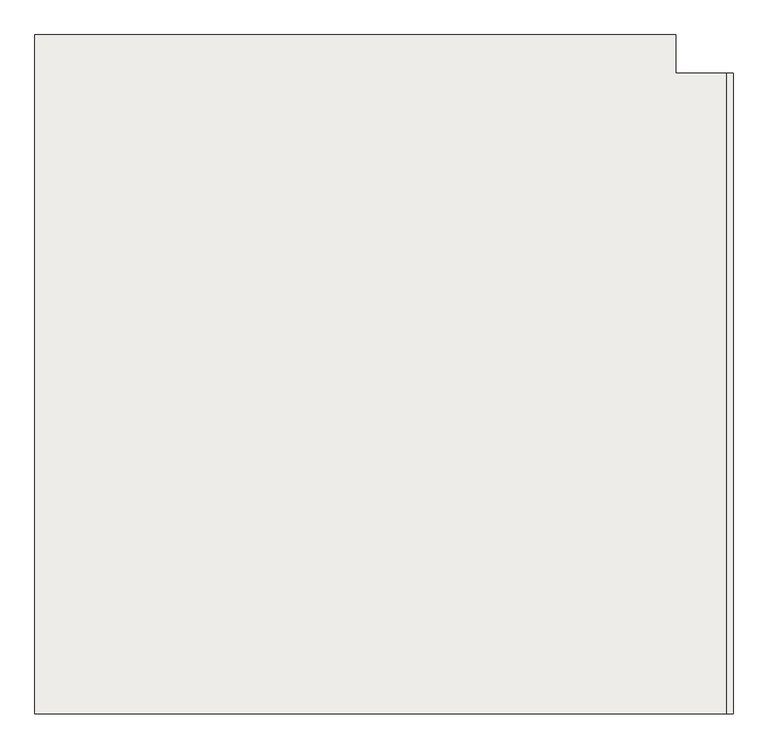
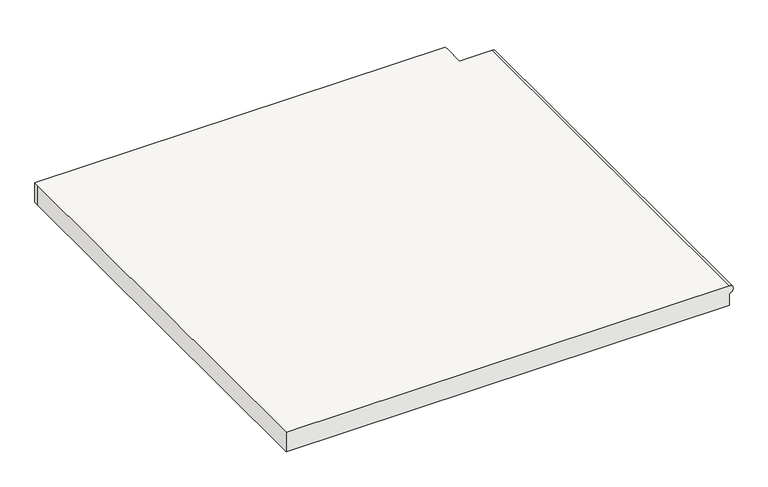
"""IFC4 building model written with IfcOpenShell, lengths in millimetres: slab geometry."""

import ifcopenshell
import ifcopenshell.guid

model = None  # the IFC model being written
_history = None  # IfcOwnerHistory: only IFC2X3 demands one
_inside = {}  # id of a spatial element -> (the spatial element, [elements in it])
_under = {}  # id of a project, library or spatial element -> (it, [spatial elements below it])
_declared = {}  # id of a project -> (the project, [libraries it declares])
_typed = {}  # id of a type object -> (the type object, [elements of that type])
_made_of = {}  # id of a material, layer set ... -> (it, [elements and type objects made of it])


def new_model(schema):
    """Start an empty IFC model of exactly this schema.

    Asked for "IFC4X3", IfcOpenShell would pick the latest addendum, in which some entities
    have other attributes; the version numbers below select the first issue.
    IFC2X3 requires an IfcOwnerHistory on every rooted entity: one is made here for all.
    """
    global model, _history
    if schema == "IFC4X3":
        model = ifcopenshell.file(schema_version=(4, 3, 0, 0))
    else:
        model = ifcopenshell.file(schema=schema)
    _inside.clear()
    _under.clear()
    _declared.clear()
    _typed.clear()
    _made_of.clear()
    _history = None
    if model.schema == "IFC2X3":
        org = make("IfcOrganization", Name="unknown")
        user = make(
            "IfcPersonAndOrganization",
            ThePerson=make("IfcPerson", FamilyName="unknown"),
            TheOrganization=org,
        )
        app = make(
            "IfcApplication",
            ApplicationDeveloper=org,
            Version="unknown",
            ApplicationFullName="unknown",
            ApplicationIdentifier="unknown",
        )
        _history = make(
            "IfcOwnerHistory",
            OwningUser=user,
            OwningApplication=app,
            ChangeAction="ADDED",
            CreationDate=0,
        )
    return model


def make(cls, **values):
    """One entity of the class cls with the attributes given. An attribute that is None is left unset."""
    return model.create_entity(
        cls, **{name: value for name, value in values.items() if value is not None}
    )


def rooted(cls, **values):
    """An entity with a GlobalId (a new one), such as an element, a storey or a relation."""
    return make(cls, GlobalId=ifcopenshell.guid.new(), OwnerHistory=_history, **values)


def si_unit(unit_type, name, prefix=None):
    """IfcSIUnit, for example si_unit("LENGTHUNIT", "METRE", prefix="MILLI")."""
    return make("IfcSIUnit", UnitType=unit_type, Prefix=prefix, Name=name)


def assignment(units):
    """IfcUnitAssignment: the units of a project."""
    return None if units is None else make("IfcUnitAssignment", Units=units)


def point(xyz):
    """IfcCartesianPoint."""
    return None if xyz is None else make("IfcCartesianPoint", Coordinates=xyz)


def direction(xyz):
    """IfcDirection."""
    return None if xyz is None else make("IfcDirection", DirectionRatios=xyz)


def frame(location, z_axis=None, x_axis=None):
    """IfcAxis2Placement3D, a coordinate frame: its origin and axes. An axis left out is left unset."""
    return make(
        "IfcAxis2Placement3D",
        Location=point(location),
        Axis=direction(z_axis),
        RefDirection=direction(x_axis),
    )


def origin():
    """The frame at (0, 0, 0) with its axes left unset."""
    return frame((0.0, 0.0, 0.0))


def place(relative_to, where):
    """IfcLocalPlacement: puts the frame where relative to a parent placement (None: the world)."""
    return make(
        "IfcLocalPlacement", PlacementRelTo=relative_to, RelativePlacement=where
    )


def context(
    kind, dimensions, precision=None, world=None, true_north=None, identifier=None
):
    """IfcGeometricRepresentationContext, for example the 3D "Model" context."""
    return make(
        "IfcGeometricRepresentationContext",
        ContextIdentifier=identifier,
        ContextType=kind,
        CoordinateSpaceDimension=dimensions,
        Precision=precision,
        WorldCoordinateSystem=world,
        TrueNorth=true_north,
    )


def project(units=None, contexts=None):
    """IfcProject with its units and contexts."""
    return rooted(
        "IfcProject",
        Name="project",
        RepresentationContexts=contexts,
        UnitsInContext=assignment(units),
    )


def spatial(cls, under=None, at=None, **own):
    """A site, building, storey or space (cls), placed at a placement, below another one or the project."""
    s = rooted(cls, ObjectPlacement=at, **own)
    if under is not None:
        _under.setdefault(under.id(), (under, []))[1].append(s)
    return s


def circle_curve(where, radius):
    """IfcCircle in the frame where."""
    return make("IfcCircle", Position=where, Radius=radius)


def shape(context_of_items, identifier, shape_type, items):
    """IfcShapeRepresentation: the items that make up one representation, for example the "Body"."""
    return make(
        "IfcShapeRepresentation",
        ContextOfItems=context_of_items,
        RepresentationIdentifier=identifier,
        RepresentationType=shape_type,
        Items=items,
    )


def source(mapping_origin, context_of_items, identifier, shape_type, items):
    """IfcRepresentationMap: a shape defined once, which mapped items show again and again."""
    return make(
        "IfcRepresentationMap",
        MappingOrigin=mapping_origin,
        MappedRepresentation=shape(context_of_items, identifier, shape_type, items),
    )


def transform(
    local_origin,
    x_axis=None,
    y_axis=None,
    z_axis=None,
    scale=None,
    scale2=None,
    scale3=None,
    uniform=True,
):
    """IfcCartesianTransformationOperator3D, or its non-uniform kind. x_axis, y_axis, z_axis: its Axis1, 2, 3."""
    if uniform:
        return make(
            "IfcCartesianTransformationOperator3D",
            Axis1=direction(x_axis),
            Axis2=direction(y_axis),
            LocalOrigin=point(local_origin),
            Scale=scale,
            Axis3=direction(z_axis),
        )
    return make(
        "IfcCartesianTransformationOperator3DnonUniform",
        Axis1=direction(x_axis),
        Axis2=direction(y_axis),
        LocalOrigin=point(local_origin),
        Scale=scale,
        Axis3=direction(z_axis),
        Scale2=scale2,
        Scale3=scale3,
    )


def mapped(mapping_source, mapping_target):
    """IfcMappedItem: shows the shape of a source again, moved by a transform."""
    return make(
        "IfcMappedItem", MappingSource=mapping_source, MappingTarget=mapping_target
    )


def made_of(thing, what):
    """Note that an element or type object is made of a material, layer set ...; save() writes the relation."""
    if what is not None:
        _made_of.setdefault(what.id(), (what, []))[1].append(thing)
    return thing


def element(
    cls,
    number,
    at=None,
    inside=None,
    cuts=None,
    type_object=None,
    material=None,
    context=None,
    identifier="Body",
    shape_type=None,
    held_by="IfcProductDefinitionShape",
    body=None,
    shapes=None,
    **own,
):
    """One element of the class cls, such as IfcWall. Its Tag is "e" and its number.

    at: its placement. inside: the storey or other place that contains it. cuts: it is an
    opening in that element (IfcRelVoidsElement). A single representation is given by context,
    identifier, shape_type and body (its items); several are given by shapes. held_by: the class
    of the entity that holds the representations. save() writes the other relations.
    """
    e = rooted(cls, Tag="e%d" % number, ObjectPlacement=at, **own)
    if body is not None:
        shapes = [shape(context, identifier, shape_type, body)]
    if shapes is not None:
        e.Representation = make(held_by, Representations=shapes)
    if inside is not None:
        _inside.setdefault(inside.id(), (inside, []))[1].append(e)
    if cuts is not None:
        rooted(
            "IfcRelVoidsElement", RelatingBuildingElement=cuts, RelatedOpeningElement=e
        )
    if type_object is not None:
        _typed.setdefault(type_object.id(), (type_object, []))[1].append(e)
    return made_of(e, material)


def aggregate(whole, parts):
    """IfcRelAggregates: a whole, such as a stair, and the parts it consists of."""
    return rooted("IfcRelAggregates", RelatingObject=whole, RelatedObjects=parts)


def save(model, path):
    """Write the relations noted so far, then the file.

    IfcRelAggregates (storeys below a building ...), IfcRelContainedInSpatialStructure (elements
    in a storey), IfcRelDefinesByType, IfcRelAssociatesMaterial and IfcRelDeclares: one each for
    every whole, place, type object, material and project.
    """
    for whole, parts in _under.values():
        aggregate(whole, parts)
    for where, things in _inside.values():
        rooted(
            "IfcRelContainedInSpatialStructure",
            RelatedElements=things,
            RelatingStructure=where,
        )
    for kind, things in _typed.values():
        rooted("IfcRelDefinesByType", RelatedObjects=things, RelatingType=kind)
    for what, things in _made_of.values():
        rooted("IfcRelAssociatesMaterial", RelatedObjects=things, RelatingMaterial=what)
    for by, libraries in _declared.values():
        rooted("IfcRelDeclares", RelatingContext=by, RelatedDefinitions=libraries)
    model.write(path)


def plane_surface(at):
    """IfcPlane: the flat surface through the origin of the frame at, square to its z axis."""
    return make("IfcPlane", Position=at)


def cylinder_surface(at, radius):
    """IfcCylindricalSurface: all points at the distance radius from the z axis of the frame at."""
    return make("IfcCylindricalSurface", Position=at, Radius=radius)


def advanced_brep(points, edges, surfaces, faces):
    """IfcAdvancedBrep: a solid bounded by faces that lie on surfaces and meet in shared edges.

    An edge is (start, end): straight between two places in points (the first is 0);
    or (start, end, curve); or (start, end, curve, False) where it runs against its curve.
    A face is (place in surfaces, loops), or (place, loops, False) where it looks against
    its surface's normal. A loop lists edges by number (the first is 1), with a minus sign
    where the edge is run from its end to its start. The first loop is the outer one.
    """
    corners = [point(p) for p in points]
    vertices = [make("IfcVertexPoint", VertexGeometry=c) for c in corners]
    made = []
    for start, end, *more in edges:
        made.append(
            make(
                "IfcEdgeCurve",
                EdgeStart=vertices[start],
                EdgeEnd=vertices[end],
                EdgeGeometry=more[0] if more else make("IfcPolyline", Points=[corners[start], corners[end]]),
                SameSense=more[1] if len(more) > 1 else True,
            )
        )
    hull = []
    for where, loops, *sense in faces:
        bounds = []
        for j, loop in enumerate(loops):
            ring = [make("IfcOrientedEdge", EdgeElement=made[abs(k) - 1], Orientation=k > 0) for k in loop]
            bounds.append(
                make(
                    "IfcFaceOuterBound" if j == 0 else "IfcFaceBound",
                    Bound=make("IfcEdgeLoop", EdgeList=ring),
                    Orientation=True,
                )
            )
        hull.append(make("IfcAdvancedFace", Bounds=bounds, FaceSurface=surfaces[where], SameSense=sense[0] if sense else True))
    return make("IfcAdvancedBrep", Outer=make("IfcClosedShell", CfsFaces=hull))


def slab_10a918a9(model_context):
    return source(origin(), model_context, "Body", "AdvancedBrep", [
        advanced_brep(
        [(-2595.8194784, -2645.3813072, 638.8235294), (-2595.8194784, -2645.3813072, 658.8235294), (-2595.8194784, -3645.3813072, 658.8235294), (-2595.8194784, -3645.3813072, 638.8235294), (-2675.5365014, -2645.3813072, 658.8235294), (-2675.5365014, -2595.3813072, 658.8235294), (-2675.5365014, -2585.3813072, 658.8235294), (-3675.5365014, -2585.3813072, 658.8235294), (-3675.5365014, -2595.3813072, 658.8235294), (-3675.5365014, -3645.3813072, 658.8235294), (-2595.8194784, -2645.3813072, 608.8235294), (-2595.8194784, -3645.3813072, 608.8235294), (-3675.5365014, -3645.3813072, 608.8235294), (-3675.5365014, -2595.3813072, 608.8235294), (-3675.5365014, -2585.3813072, 608.8235294), (-2675.5365014, -2585.3813072, 608.8235294), (-2675.5365014, -2595.3813072, 608.8235294), (-2675.5365014, -2645.3813072, 608.8235294)],
        [
            (0, 1, circle_curve(frame((-2595.8194784, -2645.3813072, 648.8235294), z_axis=(0.0, -1.0, 0.0), x_axis=(-1.0, 0.0, 0.0)), 10.0)),
            (1, 2),
            (2, 3, circle_curve(frame((-2595.8194784, -3645.3813072, 648.8235294), z_axis=(0.0, 1.0, 0.0), x_axis=(-1.0, 0.0, 0.0)), 10.0)),
            (3, 0),
            (1, 4),
            (4, 5),
            (5, 6),
            (6, 7),
            (7, 8),
            (8, 9),
            (9, 2),
            (10, 11),
            (11, 12),
            (12, 13),
            (13, 14),
            (14, 15),
            (15, 16),
            (16, 17),
            (17, 10),
            (10, 0),
            (3, 11),
            (17, 4),
            (16, 5),
            (15, 6),
            (14, 7),
            (13, 8),
            (12, 9),
        ],
        [
            cylinder_surface(frame((-2595.8194784, -2645.3813072, 648.8235294), z_axis=(0.0, 1.0, 0.0), x_axis=(-1.0, 0.0, 0.0)), 10.0),
            plane_surface(frame((-2595.8194784, -3645.3813072, 658.8235294), z_axis=(0.0, 0.0, 1.0), x_axis=(0.0, 1.0, 0.0))),
            plane_surface(frame((-2595.8194784, -3645.3813072, 608.8235294), z_axis=(0.0, 0.0, -1.0), x_axis=(0.0, -1.0, 0.0))),
            plane_surface(frame((-2595.8194784, -3645.3813072, 658.8235294), z_axis=(1.0, 0.0, 0.0), x_axis=(0.0, 0.0, -1.0))),
            plane_surface(frame((-2595.8194784, -2645.3813072, 658.8235294), z_axis=(0.0, 1.0, 0.0), x_axis=(0.0, 0.0, -1.0))),
            plane_surface(frame((-2675.5365014, -2645.3813072, 658.8235294), z_axis=(1.0, 0.0, 0.0), x_axis=(0.0, 0.0, -1.0))),
            plane_surface(frame((-2675.5365014, -2595.3813072, 658.8235294), z_axis=(1.0, 0.0, 0.0), x_axis=(0.0, 0.0, -1.0))),
            plane_surface(frame((-2675.5365014, -2585.3813072, 658.8235294), z_axis=(0.0, 1.0, 0.0), x_axis=(0.0, 0.0, -1.0))),
            plane_surface(frame((-3675.5365014, -2585.3813072, 658.8235294), z_axis=(-1.0, 0.0, 0.0), x_axis=(0.0, 0.0, -1.0))),
            plane_surface(frame((-3675.5365014, -2595.3813072, 658.8235294), z_axis=(-1.0, 0.0, 0.0), x_axis=(0.0, 0.0, -1.0))),
            plane_surface(frame((-3675.5365014, -3645.3813072, 658.8235294), z_axis=(0.0, -1.0, 0.0), x_axis=(0.0, 0.0, -1.0))),
        ],
        [
            (0, [[1, 2, 3, 4]]),
            (1, [[5, 6, 7, 8, 9, 10, 11, -2]]),
            (2, [[12, 13, 14, 15, 16, 17, 18, 19]]),
            (3, [[-12, 20, -4, 21]]),
            (4, [[-5, -1, -20, -19, 22]]),
            (5, [[-6, -22, -18, 23]]),
            (6, [[-7, -23, -17, 24]]),
            (7, [[-8, -24, -16, 25]]),
            (8, [[-9, -25, -15, 26]]),
            (9, [[-10, -26, -14, 27]]),
            (10, [[-11, -27, -13, -21, -3]]),
        ],
    ),
    ])


if __name__ == "__main__":
    model = new_model("IFC4")
    model_context = context("Model", 3, world=origin())
    ifc_project = project(units=[si_unit("LENGTHUNIT", "METRE", prefix="MILLI")], contexts=[model_context])
    site = spatial("IfcSite", under=ifc_project)
    building = spatial("IfcBuilding", under=site)
    placement = place(None, origin())
    slab_shape = slab_10a918a9(model_context)
    element("IfcSlab", 1, at=placement, inside=building, context=model_context, shape_type="MappedRepresentation", body=[
        mapped(slab_shape, transform((0.0, 0.0, 0.0), x_axis=(1.0, 0.0, 0.0), y_axis=(0.0, 1.0, 0.0), z_axis=(0.0, 0.0, 1.0))),
    ])
    save(model, "model.ifc")

# Revit data of these elements
# Element 1 (IfcSlab)
#   Materials on its faces: "Oak Flooring"
# Materials
#   "Oak Flooring": class "Wood", colour RGB 212 179 113, transparency 0, Description = "Quercus Rubra", Cost = 0
